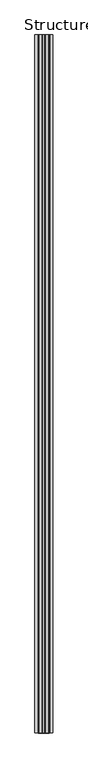
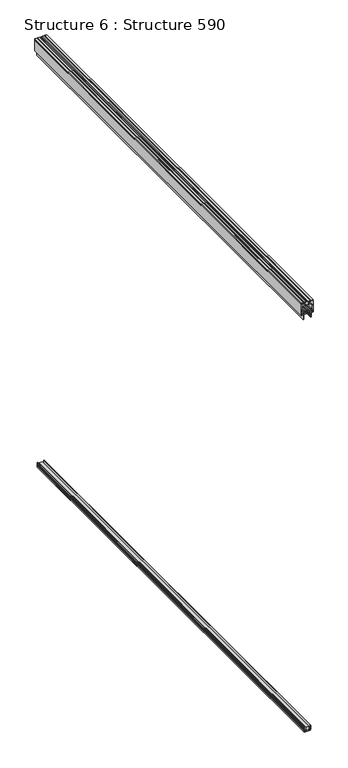
"""IFC4 building model written with IfcOpenShell, lengths in millimetres: proxy geometry, Structure 6 : Structure 590."""

from ifc_helpers import new_model, si_unit, frame, origin, place, context, project, spatial, polyline, outline, extrude, source, transform, mapped, element, save


def structure_6_structure_590_4a12d552(model_context):
    return source(origin(), model_context, "Body", "SweptSolid", [
        extrude(outline(polyline([(37604.2015618, 7622.5346434), (37604.2015618, 7648.5384455), (37606.7094313, 7651.0463151), (37611.5111794, 7651.0463151), (37613.3758754, 7650.5717441), (37616.0506024, 7651.374362), (37616.0506024, 7650.5717441), (37618.7253294, 7651.374362), (37618.7253294, 7650.5717441), (37621.4000564, 7651.374362), (37621.4000564, 7650.5717441), (37624.0747835, 7651.374362), (37624.0747835, 7650.5717441), (37626.7495105, 7650.5717441), (37628.5339519, 7648.7873027), (37606.8963912, 7648.7873027), (37606.8963912, 7642.4373027), (37609.4991896, 7642.4373027), (37609.4991896, 7628.6357862), (37606.8963912, 7628.6357862), (37606.8963912, 7622.2857862), (37628.5339519, 7622.2857862), (37626.7495105, 7620.5013448), (37624.0747835, 7620.5013448), (37624.0747835, 7619.6987269), (37621.4000564, 7620.5013448), (37621.4000564, 7619.6987269), (37618.7253294, 7620.5013448), (37618.7253294, 7619.6987269), (37616.0506024, 7620.5013448), (37616.0506024, 7619.6987269), (37613.3758754, 7620.5013448), (37611.5111794, 7620.0267738), (37606.7094313, 7620.0267738), (37604.2015618, 7622.5346434)])), frame((0.0, -3747.9491938, 0.0), z_axis=(0.0, 1.0, 0.0), x_axis=(0.0, 0.0, 1.0)), (0.0, 0.0, 1.0), 2000.0),
        extrude(outline(polyline([(7642.4373027, -3747.9491938), (7628.6357862, -3747.9491938), (7628.6357862, -1747.9491938), (7642.4373027, -1747.9491938), (7642.4373027, -3747.9491938)])), frame((0.0, 0.0, 37609.4991896), z_axis=(0.0, 0.0, 1.0), x_axis=(1.0, 0.0, 0.0)), (0.0, 0.0, 1.0), 14.5755939),
        extrude(outline(polyline([(39531.1229547, 7627.2031561), (39529.4644176, 7625.5446189), (39526.8565583, 7625.5446189), (39524.5631085, 7624.2204951), (39523.4368951, 7624.9234732), (39522.1597941, 7624.9234732), (39521.1460972, 7623.3077506), (39522.1017999, 7621.5952586), (39523.3870211, 7621.5952586), (39524.5633406, 7622.3740719), (39526.8567011, 7621.0499996), (39526.8567011, 7619.9795953), (39533.4499672, 7619.9795953), (39533.4499672, 7622.4596579), (39535.108298, 7622.4596579), (39535.108298, 7617.4647259), (39496.0572836, 7617.4647259), (39496.0572836, 7620.461166), (39498.7320107, 7620.461166), (39498.7320107, 7619.6585481), (39501.4067377, 7620.461166), (39501.4067377, 7619.6585481), (39504.0814647, 7620.461166), (39504.0814647, 7619.6585481), (39506.7561917, 7620.461166), (39506.7561917, 7619.6585481), (39509.4309187, 7620.461166), (39511.5829573, 7619.9795953), (39518.6052323, 7619.9795953), (39518.6052323, 7632.2328948), (39522.4568392, 7632.2328948), (39522.4568392, 7630.8951983), (39521.1194757, 7630.8951983), (39521.1194757, 7627.2031561), (39529.464624, 7627.2031561), (39529.464624, 7630.8951983), (39528.1272605, 7630.8951983), (39528.1272605, 7632.2049736), (39531.1229547, 7632.2049736), (39531.1229547, 7627.2031561)])), frame((0.0, -3747.9491938, 0.0), z_axis=(0.0, 1.0, 0.0), x_axis=(0.0, 0.0, 1.0)), (0.0, 0.0, 1.0), 2000.0),
        extrude(outline(polyline([(39528.1272605, 7638.8681153), (39528.1272605, 7640.1778905), (39529.464624, 7640.1778905), (39529.464624, 7643.8699328), (39521.1194757, 7643.8699328), (39521.1194757, 7640.1778905), (39522.4568392, 7640.1778905), (39522.4568392, 7638.8401941), (39518.6052323, 7638.8401941), (39518.6052323, 7651.0934936), (39511.5829573, 7651.0934936), (39509.4309187, 7650.6119229), (39506.7561917, 7651.4145408), (39506.7561917, 7650.6119229), (39504.0814647, 7651.4145408), (39504.0814647, 7650.6119229), (39501.4067377, 7651.4145408), (39501.4067377, 7650.6119229), (39498.7320107, 7651.4145408), (39498.7320107, 7650.6119229), (39496.0572836, 7650.6119229), (39496.0572836, 7653.608363), (39535.108298, 7653.608363), (39535.108298, 7648.6134309), (39533.4499672, 7648.6134309), (39533.4499672, 7651.0934936), (39526.8567011, 7651.0934936), (39526.8567011, 7650.0230892), (39524.5633406, 7648.699017), (39523.3870211, 7649.4778303), (39522.1017999, 7649.4778303), (39521.1460972, 7647.7653383), (39522.1597941, 7646.1496156), (39523.4368951, 7646.1496156), (39524.5631085, 7646.8525938), (39526.8565583, 7645.5284699), (39529.4644176, 7645.5284699), (39531.1229547, 7643.8699328), (39531.1229547, 7638.8681153), (39528.1272605, 7638.8681153)])), frame((0.0, -3747.9491938, 0.0), z_axis=(0.0, 1.0, 0.0), x_axis=(0.0, 0.0, 1.0)), (0.0, 0.0, 1.0), 2000.0),
        extrude(outline(polyline([(39569.2191527, 7660.9378957), (39572.946, 7660.9378957), (39572.946, 7653.4787112), (39570.3642897, 7653.4787112), (39571.2713147, 7652.0140696), (39570.4312008, 7650.846818), (39569.4371392, 7651.3842459), (39567.3628315, 7651.8005915), (39565.7479015, 7650.2214575), (39566.1791001, 7648.0356474), (39568.0762045, 7647.124156), (39569.7056116, 7648.1227894), (39572.946, 7648.1227894), (39572.946, 7641.2389079), (39568.7468805, 7641.2389079), (39570.179738, 7643.9279108), (39560.2371417, 7643.9279108), (39561.4571698, 7640.9834414), (39560.7401259, 7640.3771515), (39557.7331491, 7640.1428614), (39558.5286351, 7642.2701011), (39559.6684085, 7642.2701011), (39559.6684085, 7643.8442087), (39558.642991, 7643.8442087), (39558.642991, 7655.9887286), (39556.6369457, 7657.9947738), (39554.484732, 7657.9947738), (39552.7250638, 7656.9788289), (39551.5214367, 7656.9788289), (39551.5214367, 7657.9949635), (39548.8467096, 7657.9949635), (39548.8467096, 7656.9790186), (39547.643192, 7656.9790186), (39545.8835238, 7657.9949635), (39528.7060153, 7657.9949635), (39528.7060153, 7656.5234974), (39525.309112, 7656.5234974), (39525.309112, 7657.5936546), (39527.0476845, 7657.5936546), (39527.0476845, 7658.9313511), (39518.7560308, 7658.9313511), (39518.7560308, 7657.5936546), (39520.4946033, 7657.5936546), (39520.4946033, 7656.5236306), (39518.167724, 7656.5236306), (39517.0977, 7657.5936546), (39517.0977, 7660.9378957), (39565.911468, 7660.9378957), (39565.911468, 7657.3261153), (39570.9399547, 7657.3261153), (39569.2191527, 7660.9378957)])), frame((0.0, -3747.9491938, 0.0), z_axis=(0.0, 1.0, 0.0), x_axis=(0.0, 0.0, 1.0)), (0.0, 0.0, 1.0), 2000.0),
        extrude(outline(polyline([(39568.3263457, 7630.1697512), (39569.6322371, 7627.2629824), (39560.756306, 7627.2629824), (39561.8121843, 7629.5677653), (39561.8121843, 7630.4301997), (39558.6894612, 7632.8356066), (39558.6894612, 7638.3933039), (39561.7720192, 7640.7812815), (39561.7720192, 7642.0034055), (39560.819854, 7643.7400714), (39569.5290902, 7643.7400714), (39568.3928513, 7640.9829264), (39571.7499547, 7638.2793742), (39571.7499547, 7632.8582736), (39568.3263457, 7630.1697512)])), frame((0.0, -3747.9491938, 0.0), z_axis=(0.0, 1.0, 0.0), x_axis=(0.0, 0.0, 1.0)), (0.0, 0.0, 1.0), 2000.0),
        extrude(outline(polyline([(39565.911468, 7613.7469736), (39565.911468, 7610.1351931), (39517.0977, 7610.1351931), (39517.0977, 7613.4794343), (39518.167724, 7614.5494583), (39520.4946033, 7614.5494583), (39520.4946033, 7613.4794343), (39518.7560308, 7613.4794343), (39518.7560308, 7612.1417378), (39527.0476845, 7612.1417378), (39527.0476845, 7613.4794343), (39525.309112, 7613.4794343), (39525.309112, 7614.5495914), (39528.7060153, 7614.5495914), (39528.7060153, 7613.0781253), (39545.8835238, 7613.0781253), (39547.643192, 7614.0940703), (39548.8467096, 7614.0940703), (39548.8467096, 7613.0781253), (39551.5214367, 7613.0781253), (39551.5214367, 7614.09426), (39552.7250638, 7614.09426), (39554.484732, 7613.078315), (39556.6369457, 7613.078315), (39558.642991, 7615.0843603), (39558.642991, 7627.2288802), (39559.6684085, 7627.2288802), (39559.6684085, 7628.8029878), (39558.5286351, 7628.8029878), (39557.7331491, 7630.9302275), (39560.7401259, 7630.6959374), (39561.4571698, 7630.0896475), (39560.2371417, 7627.145178), (39570.179738, 7627.145178), (39568.7468805, 7629.834181), (39572.946, 7629.834181), (39572.946, 7622.9502995), (39569.7056116, 7622.9502995), (39568.0762045, 7623.9489328), (39566.1791001, 7623.0374414), (39565.7479015, 7620.8516314), (39567.3628315, 7619.2724974), (39569.4371392, 7619.688843), (39570.4312008, 7620.2262709), (39571.2713147, 7619.0590193), (39570.3642897, 7617.5943777), (39572.946, 7617.5943777), (39572.946, 7610.1351931), (39569.2191527, 7610.1351931), (39570.9399547, 7613.7469736), (39565.911468, 7613.7469736)])), frame((0.0, -3747.9491938, 0.0), z_axis=(0.0, 1.0, 0.0), x_axis=(0.0, 0.0, 1.0)), (0.0, 0.0, 1.0), 2000.0),
    ])


if __name__ == "__main__":
    model = new_model("IFC4")
    model_context = context("Model", 3, world=origin())
    ifc_project = project(units=[si_unit("LENGTHUNIT", "METRE", prefix="MILLI")], contexts=[model_context])
    site = spatial("IfcSite", under=ifc_project)
    building = spatial("IfcBuilding", under=site)
    placement = place(None, origin())
    structure_6_structure_590_shape = structure_6_structure_590_4a12d552(model_context)
    element("IfcBuildingElementProxy", 1, Name="Structure 6 : Structure 590", ObjectType="Structure 6 : Structure 590", at=placement, inside=building, context=model_context, shape_type="MappedRepresentation", body=[
        mapped(structure_6_structure_590_shape, transform((0.0, 0.0, 0.0), x_axis=(1.0, 0.0, 0.0), y_axis=(0.0, 1.0, 0.0), z_axis=(0.0, 0.0, 1.0))),
    ])
    save(model, "model.ifc")

# Revit data of these elements
# Type "Structure 6 : Structure 590"
#   NameOverride = "Structure"
# Element 1 (IfcBuildingElementProxy, "Structure 6 : Structure 590")
#   Materials on its faces: "FLEETWOOD SLIDING DOOR SERIES 3070 (SEE ELEVATIONS FOR OPERABILITY)", "RUBBER", "IfcSurfaceStyle #584"
# Materials
#   "FLEETWOOD SLIDING DOOR SERIES 3070 (SEE ELEVATIONS FOR OPERABILITY)": class "Unassigned", colour RGB 143 136 136, transparency 0, Cost = 0
#   "RUBBER": class "Unassigned", colour RGB 70 70 70, transparency 0, Cost = 0
#   "IfcSurfaceStyle #584": class "Unassigned", colour RGB 169 181 186, transparency 0
